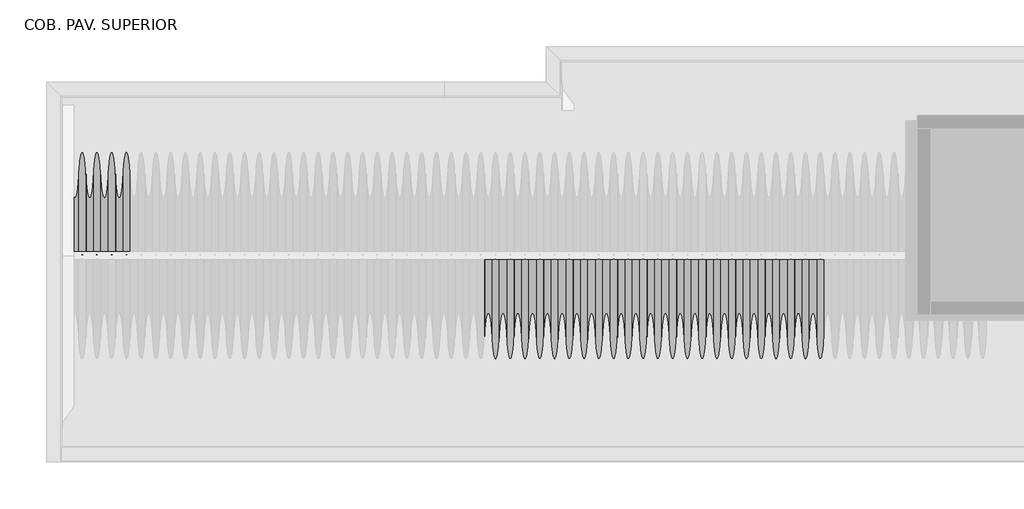
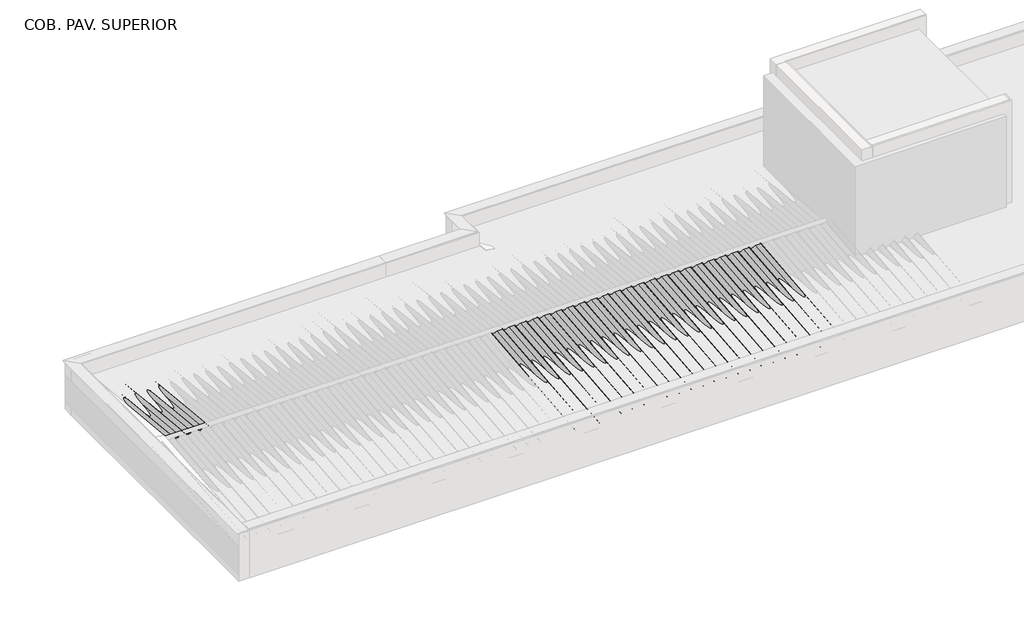
# One storey, part 3 of 8: 34 beams, 6 columns.
"""IFC4 building model written with IfcOpenShell, lengths in millimetres."""

import ifcopenshell
import ifcopenshell.guid

model = None  # the IFC model being written
_history = None  # IfcOwnerHistory: only IFC2X3 demands one
_inside = {}  # id of a spatial element -> (the spatial element, [elements in it])
_under = {}  # id of a project, library or spatial element -> (it, [spatial elements below it])
_declared = {}  # id of a project -> (the project, [libraries it declares])
_typed = {}  # id of a type object -> (the type object, [elements of that type])
_made_of = {}  # id of a material, layer set ... -> (it, [elements and type objects made of it])


def new_model(schema):
    """Start an empty IFC model of exactly this schema.

    Asked for "IFC4X3", IfcOpenShell would pick the latest addendum, in which some entities
    have other attributes; the version numbers below select the first issue.
    IFC2X3 requires an IfcOwnerHistory on every rooted entity: one is made here for all.
    """
    global model, _history
    if schema == "IFC4X3":
        model = ifcopenshell.file(schema_version=(4, 3, 0, 0))
    else:
        model = ifcopenshell.file(schema=schema)
    _inside.clear()
    _under.clear()
    _declared.clear()
    _typed.clear()
    _made_of.clear()
    _history = None
    if model.schema == "IFC2X3":
        org = make("IfcOrganization", Name="unknown")
        user = make(
            "IfcPersonAndOrganization",
            ThePerson=make("IfcPerson", FamilyName="unknown"),
            TheOrganization=org,
        )
        app = make(
            "IfcApplication",
            ApplicationDeveloper=org,
            Version="unknown",
            ApplicationFullName="unknown",
            ApplicationIdentifier="unknown",
        )
        _history = make(
            "IfcOwnerHistory",
            OwningUser=user,
            OwningApplication=app,
            ChangeAction="ADDED",
            CreationDate=0,
        )
    return model


def make(cls, **values):
    """One entity of the class cls with the attributes given. An attribute that is None is left unset."""
    return model.create_entity(
        cls, **{name: value for name, value in values.items() if value is not None}
    )


def rooted(cls, **values):
    """An entity with a GlobalId (a new one), such as an element, a storey or a relation."""
    return make(cls, GlobalId=ifcopenshell.guid.new(), OwnerHistory=_history, **values)


def si_unit(unit_type, name, prefix=None):
    """IfcSIUnit, for example si_unit("LENGTHUNIT", "METRE", prefix="MILLI")."""
    return make("IfcSIUnit", UnitType=unit_type, Prefix=prefix, Name=name)


def assignment(units):
    """IfcUnitAssignment: the units of a project."""
    return None if units is None else make("IfcUnitAssignment", Units=units)


def point(xyz):
    """IfcCartesianPoint."""
    return None if xyz is None else make("IfcCartesianPoint", Coordinates=xyz)


def direction(xyz):
    """IfcDirection."""
    return None if xyz is None else make("IfcDirection", DirectionRatios=xyz)


def frame(location, z_axis=None, x_axis=None):
    """IfcAxis2Placement3D, a coordinate frame: its origin and axes. An axis left out is left unset."""
    return make(
        "IfcAxis2Placement3D",
        Location=point(location),
        Axis=direction(z_axis),
        RefDirection=direction(x_axis),
    )


def frame_2d(location, x_axis=None):
    """IfcAxis2Placement2D, a coordinate frame in the plane: its origin and x axis."""
    return make(
        "IfcAxis2Placement2D", Location=point(location), RefDirection=direction(x_axis)
    )


def origin():
    """The frame at (0, 0, 0) with its axes left unset."""
    return frame((0.0, 0.0, 0.0))


def place(relative_to, where):
    """IfcLocalPlacement: puts the frame where relative to a parent placement (None: the world)."""
    return make(
        "IfcLocalPlacement", PlacementRelTo=relative_to, RelativePlacement=where
    )


def context(
    kind, dimensions, precision=None, world=None, true_north=None, identifier=None
):
    """IfcGeometricRepresentationContext, for example the 3D "Model" context."""
    return make(
        "IfcGeometricRepresentationContext",
        ContextIdentifier=identifier,
        ContextType=kind,
        CoordinateSpaceDimension=dimensions,
        Precision=precision,
        WorldCoordinateSystem=world,
        TrueNorth=true_north,
    )


def project(units=None, contexts=None):
    """IfcProject with its units and contexts."""
    return rooted(
        "IfcProject",
        Name="project",
        RepresentationContexts=contexts,
        UnitsInContext=assignment(units),
    )


def spatial(cls, under=None, at=None, **own):
    """A site, building, storey or space (cls), placed at a placement, below another one or the project."""
    s = rooted(cls, ObjectPlacement=at, **own)
    if under is not None:
        _under.setdefault(under.id(), (under, []))[1].append(s)
    return s


def polyline(points):
    """IfcPolyline through the points."""
    return make("IfcPolyline", Points=[point(p) for p in points])


def circle_curve(where, radius):
    """IfcCircle in the frame where."""
    return make("IfcCircle", Position=where, Radius=radius)


def trimmed(basis, trim1, trim2, sense, master):
    """IfcTrimmedCurve: the piece of a basis curve between two trims."""
    return make(
        "IfcTrimmedCurve",
        BasisCurve=basis,
        Trim1=trim1,
        Trim2=trim2,
        SenseAgreement=sense,
        MasterRepresentation=master,
    )


def segment(curve, same_sense, transition):
    """IfcCompositeCurveSegment."""
    return make(
        "IfcCompositeCurveSegment",
        Transition=transition,
        SameSense=same_sense,
        ParentCurve=curve,
    )


def composite_curve(segments, self_intersect=None):
    """IfcCompositeCurve: segments joined end to end."""
    return make("IfcCompositeCurve", Segments=segments, SelfIntersect=self_intersect)


def outline(outer, holes=None, kind="AREA"):
    """IfcArbitraryClosedProfileDef: a profile drawn as a closed curve; with holes, ...WithVoids."""
    if holes is None:
        return make("IfcArbitraryClosedProfileDef", ProfileType=kind, OuterCurve=outer)
    return make(
        "IfcArbitraryProfileDefWithVoids",
        ProfileType=kind,
        OuterCurve=outer,
        InnerCurves=holes,
    )


def extrude(swept, where, along, depth):
    """IfcExtrudedAreaSolid: the profile swept, set in the frame where, extruded along a direction by depth."""
    return make(
        "IfcExtrudedAreaSolid",
        SweptArea=swept,
        Position=where,
        ExtrudedDirection=direction(along),
        Depth=depth,
    )


def shape(context_of_items, identifier, shape_type, items):
    """IfcShapeRepresentation: the items that make up one representation, for example the "Body"."""
    return make(
        "IfcShapeRepresentation",
        ContextOfItems=context_of_items,
        RepresentationIdentifier=identifier,
        RepresentationType=shape_type,
        Items=items,
    )


def source(mapping_origin, context_of_items, identifier, shape_type, items):
    """IfcRepresentationMap: a shape defined once, which mapped items show again and again."""
    return make(
        "IfcRepresentationMap",
        MappingOrigin=mapping_origin,
        MappedRepresentation=shape(context_of_items, identifier, shape_type, items),
    )


def transform(
    local_origin,
    x_axis=None,
    y_axis=None,
    z_axis=None,
    scale=None,
    scale2=None,
    scale3=None,
    uniform=True,
):
    """IfcCartesianTransformationOperator3D, or its non-uniform kind. x_axis, y_axis, z_axis: its Axis1, 2, 3."""
    if uniform:
        return make(
            "IfcCartesianTransformationOperator3D",
            Axis1=direction(x_axis),
            Axis2=direction(y_axis),
            LocalOrigin=point(local_origin),
            Scale=scale,
            Axis3=direction(z_axis),
        )
    return make(
        "IfcCartesianTransformationOperator3DnonUniform",
        Axis1=direction(x_axis),
        Axis2=direction(y_axis),
        LocalOrigin=point(local_origin),
        Scale=scale,
        Axis3=direction(z_axis),
        Scale2=scale2,
        Scale3=scale3,
    )


def mapped(mapping_source, mapping_target):
    """IfcMappedItem: shows the shape of a source again, moved by a transform."""
    return make(
        "IfcMappedItem", MappingSource=mapping_source, MappingTarget=mapping_target
    )


def made_of(thing, what):
    """Note that an element or type object is made of a material, layer set ...; save() writes the relation."""
    if what is not None:
        _made_of.setdefault(what.id(), (what, []))[1].append(thing)
    return thing


def element(
    cls,
    number,
    at=None,
    inside=None,
    cuts=None,
    type_object=None,
    material=None,
    context=None,
    identifier="Body",
    shape_type=None,
    held_by="IfcProductDefinitionShape",
    body=None,
    shapes=None,
    **own,
):
    """One element of the class cls, such as IfcWall. Its Tag is "e" and its number.

    at: its placement. inside: the storey or other place that contains it. cuts: it is an
    opening in that element (IfcRelVoidsElement). A single representation is given by context,
    identifier, shape_type and body (its items); several are given by shapes. held_by: the class
    of the entity that holds the representations. save() writes the other relations.
    """
    e = rooted(cls, Tag="e%d" % number, ObjectPlacement=at, **own)
    if body is not None:
        shapes = [shape(context, identifier, shape_type, body)]
    if shapes is not None:
        e.Representation = make(held_by, Representations=shapes)
    if inside is not None:
        _inside.setdefault(inside.id(), (inside, []))[1].append(e)
    if cuts is not None:
        rooted(
            "IfcRelVoidsElement", RelatingBuildingElement=cuts, RelatedOpeningElement=e
        )
    if type_object is not None:
        _typed.setdefault(type_object.id(), (type_object, []))[1].append(e)
    return made_of(e, material)


def aggregate(whole, parts):
    """IfcRelAggregates: a whole, such as a stair, and the parts it consists of."""
    return rooted("IfcRelAggregates", RelatingObject=whole, RelatedObjects=parts)


def save(model, path):
    """Write the relations noted so far, then the file.

    IfcRelAggregates (storeys below a building ...), IfcRelContainedInSpatialStructure (elements
    in a storey), IfcRelDefinesByType, IfcRelAssociatesMaterial and IfcRelDeclares: one each for
    every whole, place, type object, material and project.
    """
    for whole, parts in _under.values():
        aggregate(whole, parts)
    for where, things in _inside.values():
        rooted(
            "IfcRelContainedInSpatialStructure",
            RelatedElements=things,
            RelatingStructure=where,
        )
    for kind, things in _typed.values():
        rooted("IfcRelDefinesByType", RelatedObjects=things, RelatingType=kind)
    for what, things in _made_of.values():
        rooted("IfcRelAssociatesMaterial", RelatedObjects=things, RelatingMaterial=what)
    for by, libraries in _declared.values():
        rooted("IfcRelDeclares", RelatingContext=by, RelatedDefinitions=libraries)
    model.write(path)


def beam_fe4ddbad(model_context):
    return source(origin(), model_context, "Body", "SweptSolid", [
        extrude(outline(polyline([(998.8971968, 30.0), (998.8971968, -30.0), (-998.8971974, -30.0), (-998.8971974, 30.0), (998.8971968, 30.0)])), frame((0.0, 0.0, -60.0), z_axis=(0.0, 0.0, 1.0), x_axis=(1.0, 0.0, 0.0)), (0.0, 0.0, 1.0), 120.0),
    ])


def column_6c15bf79(model_context):
    return source(origin(), model_context, "Body", "SweptSolid", [
        extrude(outline(polyline([(30.0, 80.0), (30.0, -80.0), (-30.0, -80.0), (-30.0, 80.0), (30.0, 80.0)])), frame((0.0, 0.0, 6710.0), z_axis=(0.0, 0.0, 1.0), x_axis=(1.0, 0.0, 0.0)), (0.0, 0.0, 1.0), 467.5),
    ])


def column_42eef9f8(model_context):
    return source(origin(), model_context, "Body", "SweptSolid", [
        extrude(outline(polyline([(30.0, 80.0), (30.0, -80.0), (-30.0, -80.0), (-30.0, 80.0), (30.0, 80.0)])), frame((0.0, 0.0, 6710.0), z_axis=(0.0, 0.0, 1.0), x_axis=(1.0, 0.0, 0.0)), (0.0, 0.0, 1.0), 227.1),
    ])


model = new_model("IFC4")

# Units and contexts
model_context = context("Model", 3, world=origin())
ifc_project = project(units=[si_unit("LENGTHUNIT", "METRE", prefix="MILLI")], contexts=[model_context])

# Site, building, storey
site = spatial("IfcSite", under=ifc_project)
building = spatial("IfcBuilding", under=site)
storey = spatial("IfcBuildingStorey", under=building, Name="COB. PAV. SUPERIOR", Elevation=6650.0)

# Beams
placement = place(None, origin())
beam_shape = beam_fe4ddbad(model_context)
element("IfcBeam", 1, ObjectType="Madeira de lei : Berço 6x12cm", at=placement, inside=storey, context=model_context, shape_type="MappedRepresentation", body=[
    mapped(beam_shape, transform((-11738.1841096, -7777.6209418, 6680.0), x_axis=(1.0, 0.0, 0.0), y_axis=(0.0, 0.0, -1.0), z_axis=(0.0, 1.0, 0.0))),
])
element("IfcBeam", 2, ObjectType="Madeira de lei : Berço 6x12cm", at=placement, inside=storey, context=model_context, shape_type="MappedRepresentation", body=[
    mapped(beam_shape, transform((-5744.8009251, -9189.768869, 6680.0), x_axis=(1.0, 0.0, 0.0), y_axis=(0.0, 0.0, -1.0), z_axis=(0.0, 1.0, 0.0))),
])
element("IfcBeam", 3, ObjectType="Madeira de lei : Berço 6x12cm", at=placement, inside=storey, context=model_context, shape_type="MappedRepresentation", body=[
    mapped(beam_shape, transform((-3747.0065303, -9189.768869, 6680.0), x_axis=(1.0, 0.0, 0.0), y_axis=(0.0, 0.0, -1.0), z_axis=(0.0, 1.0, 0.0))),
])
element("IfcBeam", 4, ObjectType="Madeira de lei : Berço 6x12cm", at=placement, inside=storey, context=model_context, shape_type="MappedRepresentation", body=[
    mapped(beam_shape, transform((-1749.2121355, -9189.768869, 6680.0), x_axis=(1.0, 0.0, 0.0), y_axis=(0.0, 0.0, -1.0), z_axis=(0.0, 1.0, 0.0))),
])
element("IfcBeam", 5, ObjectType="Madeira de lei : Berço 6x12cm", at=placement, inside=storey, context=model_context, shape_type="MappedRepresentation", body=[
    mapped(beam_shape, transform((-3747.0065303, -10631.818869, 6680.0), x_axis=(1.0, 0.0, 0.0), y_axis=(0.0, 0.0, -1.0), z_axis=(0.0, 1.0, 0.0))),
])
element("IfcBeam", 6, ObjectType="Madeira de lei : Berço 6x12cm", at=placement, inside=storey, context=model_context, shape_type="MappedRepresentation", body=[
    mapped(beam_shape, transform((-1749.2121355, -10631.818869, 6680.0), x_axis=(1.0, 0.0, 0.0), y_axis=(0.0, 0.0, -1.0), z_axis=(0.0, 1.0, 0.0))),
])
element("IfcBeam", 7, ObjectType="Telha Ondulada : Fibrocimento", at=placement, inside=storey, context=model_context, shape_type="SweptSolid", body=[
    extrude(outline(composite_curve([segment(trimmed(circle_curve(frame_2d((0.0, 66.7939461)), 66.7939461), [point((29.3501489, 6.7939461))], [point((29.3501489, 126.7939461))], True, "CARTESIAN"), True, "CONTINUOUS"), segment(polyline([(29.3501489, 126.7939461), (31.5472154, 131.2853711)]), True, "CONTINUOUS"), segment(trimmed(circle_curve(frame_2d((0.0, 66.7939461)), 71.7939461), [point((31.5472154, 131.2853711))], [point((31.5472154, 2.3025211))], False, "CARTESIAN"), True, "CONTINUOUS"), segment(trimmed(circle_curve(frame_2d((58.7002978, -53.2060539)), 61.7939461), [point((31.5472154, 2.3025211))], [point((31.5472154, -108.7146289))], True, "CARTESIAN"), True, "CONTINUOUS"), segment(polyline([(31.5472154, -108.7146289), (29.3501489, -113.2060539)]), True, "CONTINUOUS"), segment(trimmed(circle_curve(frame_2d((58.7002978, -53.2060539)), 66.7939461), [point((29.3501489, -113.2060539))], [point((29.3501489, 6.7939461))], False, "CARTESIAN"), True, "CONTINUOUS")], self_intersect=False)), frame((-5606.7843743, -10831.9594023, 7106.8215886), z_axis=(0.0, 0.9950371902099894, 0.09950371902099749), x_axis=(0.0, 0.09950371902099749, -0.9950371902099894)), (0.0, 0.0, 1.0), 3060.4439799),
])
element("IfcBeam", 8, ObjectType="Telha Ondulada : Fibrocimento", at=placement, inside=storey, context=model_context, shape_type="SweptSolid", body=[
    extrude(outline(composite_curve([segment(trimmed(circle_curve(frame_2d((0.0, 66.7939461)), 66.7939461), [point((29.3501489, 6.7939461))], [point((29.3501489, 126.7939461))], True, "CARTESIAN"), True, "CONTINUOUS"), segment(polyline([(29.3501489, 126.7939461), (31.5472154, 131.2853711)]), True, "CONTINUOUS"), segment(trimmed(circle_curve(frame_2d((0.0, 66.7939461)), 71.7939461), [point((31.5472154, 131.2853711))], [point((31.5472154, 2.3025211))], False, "CARTESIAN"), True, "CONTINUOUS"), segment(trimmed(circle_curve(frame_2d((58.7002978, -53.2060539)), 61.7939461), [point((31.5472154, 2.3025211))], [point((31.5472154, -108.7146289))], True, "CARTESIAN"), True, "CONTINUOUS"), segment(polyline([(31.5472154, -108.7146289), (29.3501489, -113.2060539)]), True, "CONTINUOUS"), segment(trimmed(circle_curve(frame_2d((58.7002978, -53.2060539)), 66.7939461), [point((29.3501489, -113.2060539))], [point((29.3501489, 6.7939461))], False, "CARTESIAN"), True, "CONTINUOUS")], self_intersect=False)), frame((-5362.2843743, -10831.9594023, 7106.8215886), z_axis=(0.0, 0.9950371902099894, 0.09950371902099749), x_axis=(0.0, 0.09950371902099749, -0.9950371902099894)), (0.0, 0.0, 1.0), 3060.4439799),
])
element("IfcBeam", 9, ObjectType="Telha Ondulada : Fibrocimento", at=placement, inside=storey, context=model_context, shape_type="SweptSolid", body=[
    extrude(outline(composite_curve([segment(trimmed(circle_curve(frame_2d((0.0, 66.7939461)), 66.7939461), [point((29.3501489, 6.7939461))], [point((29.3501489, 126.7939461))], True, "CARTESIAN"), True, "CONTINUOUS"), segment(polyline([(29.3501489, 126.7939461), (31.5472154, 131.2853711)]), True, "CONTINUOUS"), segment(trimmed(circle_curve(frame_2d((0.0, 66.7939461)), 71.7939461), [point((31.5472154, 131.2853711))], [point((31.5472154, 2.3025211))], False, "CARTESIAN"), True, "CONTINUOUS"), segment(trimmed(circle_curve(frame_2d((58.7002978, -53.2060539)), 61.7939461), [point((31.5472154, 2.3025211))], [point((31.5472154, -108.7146289))], True, "CARTESIAN"), True, "CONTINUOUS"), segment(polyline([(31.5472154, -108.7146289), (29.3501489, -113.2060539)]), True, "CONTINUOUS"), segment(trimmed(circle_curve(frame_2d((58.7002978, -53.2060539)), 66.7939461), [point((29.3501489, -113.2060539))], [point((29.3501489, 6.7939461))], False, "CARTESIAN"), True, "CONTINUOUS")], self_intersect=False)), frame((-5117.7843743, -10831.9594023, 7106.8215886), z_axis=(0.0, 0.9950371902099894, 0.09950371902099749), x_axis=(0.0, 0.09950371902099749, -0.9950371902099894)), (0.0, 0.0, 1.0), 3060.4439799),
])
element("IfcBeam", 10, ObjectType="Telha Ondulada : Fibrocimento", at=placement, inside=storey, context=model_context, shape_type="SweptSolid", body=[
    extrude(outline(composite_curve([segment(trimmed(circle_curve(frame_2d((0.0, 66.7939461)), 66.7939461), [point((29.3501489, 6.7939461))], [point((29.3501489, 126.7939461))], True, "CARTESIAN"), True, "CONTINUOUS"), segment(polyline([(29.3501489, 126.7939461), (31.5472154, 131.2853711)]), True, "CONTINUOUS"), segment(trimmed(circle_curve(frame_2d((0.0, 66.7939461)), 71.7939461), [point((31.5472154, 131.2853711))], [point((31.5472154, 2.3025211))], False, "CARTESIAN"), True, "CONTINUOUS"), segment(trimmed(circle_curve(frame_2d((58.7002978, -53.2060539)), 61.7939461), [point((31.5472154, 2.3025211))], [point((31.5472154, -108.7146289))], True, "CARTESIAN"), True, "CONTINUOUS"), segment(polyline([(31.5472154, -108.7146289), (29.3501489, -113.2060539)]), True, "CONTINUOUS"), segment(trimmed(circle_curve(frame_2d((58.7002978, -53.2060539)), 66.7939461), [point((29.3501489, -113.2060539))], [point((29.3501489, 6.7939461))], False, "CARTESIAN"), True, "CONTINUOUS")], self_intersect=False)), frame((-4873.2843743, -10831.9594023, 7106.8215886), z_axis=(0.0, 0.9950371902099894, 0.09950371902099749), x_axis=(0.0, 0.09950371902099749, -0.9950371902099894)), (0.0, 0.0, 1.0), 3060.4439799),
])
element("IfcBeam", 11, ObjectType="Telha Ondulada : Fibrocimento", at=placement, inside=storey, context=model_context, shape_type="SweptSolid", body=[
    extrude(outline(composite_curve([segment(trimmed(circle_curve(frame_2d((0.0, 66.7939461)), 66.7939461), [point((29.3501489, 6.7939461))], [point((29.3501489, 126.7939461))], True, "CARTESIAN"), True, "CONTINUOUS"), segment(polyline([(29.3501489, 126.7939461), (31.5472154, 131.2853711)]), True, "CONTINUOUS"), segment(trimmed(circle_curve(frame_2d((0.0, 66.7939461)), 71.7939461), [point((31.5472154, 131.2853711))], [point((31.5472154, 2.3025211))], False, "CARTESIAN"), True, "CONTINUOUS"), segment(trimmed(circle_curve(frame_2d((58.7002978, -53.2060539)), 61.7939461), [point((31.5472154, 2.3025211))], [point((31.5472154, -108.7146289))], True, "CARTESIAN"), True, "CONTINUOUS"), segment(polyline([(31.5472154, -108.7146289), (29.3501489, -113.2060539)]), True, "CONTINUOUS"), segment(trimmed(circle_curve(frame_2d((58.7002978, -53.2060539)), 66.7939461), [point((29.3501489, -113.2060539))], [point((29.3501489, 6.7939461))], False, "CARTESIAN"), True, "CONTINUOUS")], self_intersect=False)), frame((-4628.7843743, -10831.9594023, 7106.8215886), z_axis=(0.0, 0.9950371902099894, 0.09950371902099749), x_axis=(0.0, 0.09950371902099749, -0.9950371902099894)), (0.0, 0.0, 1.0), 3060.4439799),
])
element("IfcBeam", 12, ObjectType="Telha Ondulada : Fibrocimento", at=placement, inside=storey, context=model_context, shape_type="SweptSolid", body=[
    extrude(outline(composite_curve([segment(trimmed(circle_curve(frame_2d((0.0, 66.7939461)), 66.7939461), [point((29.3501489, 6.7939461))], [point((29.3501489, 126.7939461))], True, "CARTESIAN"), True, "CONTINUOUS"), segment(polyline([(29.3501489, 126.7939461), (31.5472154, 131.2853711)]), True, "CONTINUOUS"), segment(trimmed(circle_curve(frame_2d((0.0, 66.7939461)), 71.7939461), [point((31.5472154, 131.2853711))], [point((31.5472154, 2.3025211))], False, "CARTESIAN"), True, "CONTINUOUS"), segment(trimmed(circle_curve(frame_2d((58.7002978, -53.2060539)), 61.7939461), [point((31.5472154, 2.3025211))], [point((31.5472154, -108.7146289))], True, "CARTESIAN"), True, "CONTINUOUS"), segment(polyline([(31.5472154, -108.7146289), (29.3501489, -113.2060539)]), True, "CONTINUOUS"), segment(trimmed(circle_curve(frame_2d((58.7002978, -53.2060539)), 66.7939461), [point((29.3501489, -113.2060539))], [point((29.3501489, 6.7939461))], False, "CARTESIAN"), True, "CONTINUOUS")], self_intersect=False)), frame((-4384.2843743, -10831.9594023, 7106.8215886), z_axis=(0.0, 0.9950371902099894, 0.09950371902099749), x_axis=(0.0, 0.09950371902099749, -0.9950371902099894)), (0.0, 0.0, 1.0), 3060.4439799),
])
element("IfcBeam", 13, ObjectType="Telha Ondulada : Fibrocimento", at=placement, inside=storey, context=model_context, shape_type="SweptSolid", body=[
    extrude(outline(composite_curve([segment(trimmed(circle_curve(frame_2d((0.0, 66.7939461)), 66.7939461), [point((29.3501489, 6.7939461))], [point((29.3501489, 126.7939461))], True, "CARTESIAN"), True, "CONTINUOUS"), segment(polyline([(29.3501489, 126.7939461), (31.5472154, 131.2853711)]), True, "CONTINUOUS"), segment(trimmed(circle_curve(frame_2d((0.0, 66.7939461)), 71.7939461), [point((31.5472154, 131.2853711))], [point((31.5472154, 2.3025211))], False, "CARTESIAN"), True, "CONTINUOUS"), segment(trimmed(circle_curve(frame_2d((58.7002978, -53.2060539)), 61.7939461), [point((31.5472154, 2.3025211))], [point((31.5472154, -108.7146289))], True, "CARTESIAN"), True, "CONTINUOUS"), segment(polyline([(31.5472154, -108.7146289), (29.3501489, -113.2060539)]), True, "CONTINUOUS"), segment(trimmed(circle_curve(frame_2d((58.7002978, -53.2060539)), 66.7939461), [point((29.3501489, -113.2060539))], [point((29.3501489, 6.7939461))], False, "CARTESIAN"), True, "CONTINUOUS")], self_intersect=False)), frame((-4139.7843743, -10831.9594023, 7106.8215886), z_axis=(0.0, 0.9950371902099894, 0.09950371902099749), x_axis=(0.0, 0.09950371902099749, -0.9950371902099894)), (0.0, 0.0, 1.0), 3060.4439799),
])
element("IfcBeam", 14, ObjectType="Telha Ondulada : Fibrocimento", at=placement, inside=storey, context=model_context, shape_type="SweptSolid", body=[
    extrude(outline(composite_curve([segment(trimmed(circle_curve(frame_2d((0.0, 66.7939461)), 66.7939461), [point((29.3501489, 6.7939461))], [point((29.3501489, 126.7939461))], True, "CARTESIAN"), True, "CONTINUOUS"), segment(polyline([(29.3501489, 126.7939461), (31.5472154, 131.2853711)]), True, "CONTINUOUS"), segment(trimmed(circle_curve(frame_2d((0.0, 66.7939461)), 71.7939461), [point((31.5472154, 131.2853711))], [point((31.5472154, 2.3025211))], False, "CARTESIAN"), True, "CONTINUOUS"), segment(trimmed(circle_curve(frame_2d((58.7002978, -53.2060539)), 61.7939461), [point((31.5472154, 2.3025211))], [point((31.5472154, -108.7146289))], True, "CARTESIAN"), True, "CONTINUOUS"), segment(polyline([(31.5472154, -108.7146289), (29.3501489, -113.2060539)]), True, "CONTINUOUS"), segment(trimmed(circle_curve(frame_2d((58.7002978, -53.2060539)), 66.7939461), [point((29.3501489, -113.2060539))], [point((29.3501489, 6.7939461))], False, "CARTESIAN"), True, "CONTINUOUS")], self_intersect=False)), frame((-3895.2843743, -10831.9594023, 7106.8215886), z_axis=(0.0, 0.9950371902099894, 0.09950371902099749), x_axis=(0.0, 0.09950371902099749, -0.9950371902099894)), (0.0, 0.0, 1.0), 3060.4439799),
])
element("IfcBeam", 15, ObjectType="Telha Ondulada : Fibrocimento", at=placement, inside=storey, context=model_context, shape_type="SweptSolid", body=[
    extrude(outline(composite_curve([segment(trimmed(circle_curve(frame_2d((0.0, 66.7939461)), 66.7939461), [point((29.3501489, 6.7939461))], [point((29.3501489, 126.7939461))], True, "CARTESIAN"), True, "CONTINUOUS"), segment(polyline([(29.3501489, 126.7939461), (31.5472154, 131.2853711)]), True, "CONTINUOUS"), segment(trimmed(circle_curve(frame_2d((0.0, 66.7939461)), 71.7939461), [point((31.5472154, 131.2853711))], [point((31.5472154, 2.3025211))], False, "CARTESIAN"), True, "CONTINUOUS"), segment(trimmed(circle_curve(frame_2d((58.7002978, -53.2060539)), 61.7939461), [point((31.5472154, 2.3025211))], [point((31.5472154, -108.7146289))], True, "CARTESIAN"), True, "CONTINUOUS"), segment(polyline([(31.5472154, -108.7146289), (29.3501489, -113.2060539)]), True, "CONTINUOUS"), segment(trimmed(circle_curve(frame_2d((58.7002978, -53.2060539)), 66.7939461), [point((29.3501489, -113.2060539))], [point((29.3501489, 6.7939461))], False, "CARTESIAN"), True, "CONTINUOUS")], self_intersect=False)), frame((-3650.7843743, -10831.9594023, 7106.8215886), z_axis=(0.0, 0.9950371902099894, 0.09950371902099749), x_axis=(0.0, 0.09950371902099749, -0.9950371902099894)), (0.0, 0.0, 1.0), 3060.4439799),
])
element("IfcBeam", 16, ObjectType="Telha Ondulada : Fibrocimento", at=placement, inside=storey, context=model_context, shape_type="SweptSolid", body=[
    extrude(outline(composite_curve([segment(trimmed(circle_curve(frame_2d((0.0, 66.7939461)), 66.7939461), [point((29.3501489, 6.7939461))], [point((29.3501489, 126.7939461))], True, "CARTESIAN"), True, "CONTINUOUS"), segment(polyline([(29.3501489, 126.7939461), (31.5472154, 131.2853711)]), True, "CONTINUOUS"), segment(trimmed(circle_curve(frame_2d((0.0, 66.7939461)), 71.7939461), [point((31.5472154, 131.2853711))], [point((31.5472154, 2.3025211))], False, "CARTESIAN"), True, "CONTINUOUS"), segment(trimmed(circle_curve(frame_2d((58.7002978, -53.2060539)), 61.7939461), [point((31.5472154, 2.3025211))], [point((31.5472154, -108.7146289))], True, "CARTESIAN"), True, "CONTINUOUS"), segment(polyline([(31.5472154, -108.7146289), (29.3501489, -113.2060539)]), True, "CONTINUOUS"), segment(trimmed(circle_curve(frame_2d((58.7002978, -53.2060539)), 66.7939461), [point((29.3501489, -113.2060539))], [point((29.3501489, 6.7939461))], False, "CARTESIAN"), True, "CONTINUOUS")], self_intersect=False)), frame((-3406.2843743, -10831.9594023, 7106.8215886), z_axis=(0.0, 0.9950371902099894, 0.09950371902099749), x_axis=(0.0, 0.09950371902099749, -0.9950371902099894)), (0.0, 0.0, 1.0), 3060.4439799),
])
element("IfcBeam", 17, ObjectType="Telha Ondulada : Fibrocimento", at=placement, inside=storey, context=model_context, shape_type="SweptSolid", body=[
    extrude(outline(composite_curve([segment(trimmed(circle_curve(frame_2d((0.0, 66.7939461)), 66.7939461), [point((29.3501489, 6.7939461))], [point((29.3501489, 126.7939461))], True, "CARTESIAN"), True, "CONTINUOUS"), segment(polyline([(29.3501489, 126.7939461), (31.5472154, 131.2853711)]), True, "CONTINUOUS"), segment(trimmed(circle_curve(frame_2d((0.0, 66.7939461)), 71.7939461), [point((31.5472154, 131.2853711))], [point((31.5472154, 2.3025211))], False, "CARTESIAN"), True, "CONTINUOUS"), segment(trimmed(circle_curve(frame_2d((58.7002978, -53.2060539)), 61.7939461), [point((31.5472154, 2.3025211))], [point((31.5472154, -108.7146289))], True, "CARTESIAN"), True, "CONTINUOUS"), segment(polyline([(31.5472154, -108.7146289), (29.3501489, -113.2060539)]), True, "CONTINUOUS"), segment(trimmed(circle_curve(frame_2d((58.7002978, -53.2060539)), 66.7939461), [point((29.3501489, -113.2060539))], [point((29.3501489, 6.7939461))], False, "CARTESIAN"), True, "CONTINUOUS")], self_intersect=False)), frame((-3161.7843743, -10831.9594023, 7106.8215886), z_axis=(0.0, 0.9950371902099894, 0.09950371902099749), x_axis=(0.0, 0.09950371902099749, -0.9950371902099894)), (0.0, 0.0, 1.0), 3060.4439799),
])
element("IfcBeam", 18, ObjectType="Telha Ondulada : Fibrocimento", at=placement, inside=storey, context=model_context, shape_type="SweptSolid", body=[
    extrude(outline(composite_curve([segment(trimmed(circle_curve(frame_2d((0.0, 66.7939461)), 66.7939461), [point((29.3501489, 6.7939461))], [point((29.3501489, 126.7939461))], True, "CARTESIAN"), True, "CONTINUOUS"), segment(polyline([(29.3501489, 126.7939461), (31.5472154, 131.2853711)]), True, "CONTINUOUS"), segment(trimmed(circle_curve(frame_2d((0.0, 66.7939461)), 71.7939461), [point((31.5472154, 131.2853711))], [point((31.5472154, 2.3025211))], False, "CARTESIAN"), True, "CONTINUOUS"), segment(trimmed(circle_curve(frame_2d((58.7002978, -53.2060539)), 61.7939461), [point((31.5472154, 2.3025211))], [point((31.5472154, -108.7146289))], True, "CARTESIAN"), True, "CONTINUOUS"), segment(polyline([(31.5472154, -108.7146289), (29.3501489, -113.2060539)]), True, "CONTINUOUS"), segment(trimmed(circle_curve(frame_2d((58.7002978, -53.2060539)), 66.7939461), [point((29.3501489, -113.2060539))], [point((29.3501489, 6.7939461))], False, "CARTESIAN"), True, "CONTINUOUS")], self_intersect=False)), frame((-2917.2843743, -10831.9594023, 7106.8215886), z_axis=(0.0, 0.9950371902099894, 0.09950371902099749), x_axis=(0.0, 0.09950371902099749, -0.9950371902099894)), (0.0, 0.0, 1.0), 3060.4439799),
])
element("IfcBeam", 19, ObjectType="Telha Ondulada : Fibrocimento", at=placement, inside=storey, context=model_context, shape_type="SweptSolid", body=[
    extrude(outline(composite_curve([segment(trimmed(circle_curve(frame_2d((0.0, 66.7939461)), 66.7939461), [point((29.3501489, 6.7939461))], [point((29.3501489, 126.7939461))], True, "CARTESIAN"), True, "CONTINUOUS"), segment(polyline([(29.3501489, 126.7939461), (31.5472154, 131.2853711)]), True, "CONTINUOUS"), segment(trimmed(circle_curve(frame_2d((0.0, 66.7939461)), 71.7939461), [point((31.5472154, 131.2853711))], [point((31.5472154, 2.3025211))], False, "CARTESIAN"), True, "CONTINUOUS"), segment(trimmed(circle_curve(frame_2d((58.7002978, -53.2060539)), 61.7939461), [point((31.5472154, 2.3025211))], [point((31.5472154, -108.7146289))], True, "CARTESIAN"), True, "CONTINUOUS"), segment(polyline([(31.5472154, -108.7146289), (29.3501489, -113.2060539)]), True, "CONTINUOUS"), segment(trimmed(circle_curve(frame_2d((58.7002978, -53.2060539)), 66.7939461), [point((29.3501489, -113.2060539))], [point((29.3501489, 6.7939461))], False, "CARTESIAN"), True, "CONTINUOUS")], self_intersect=False)), frame((-2672.7843743, -10831.9594023, 7106.8215886), z_axis=(0.0, 0.9950371902099894, 0.09950371902099749), x_axis=(0.0, 0.09950371902099749, -0.9950371902099894)), (0.0, 0.0, 1.0), 3060.4439799),
])
element("IfcBeam", 20, ObjectType="Telha Ondulada : Fibrocimento", at=placement, inside=storey, context=model_context, shape_type="SweptSolid", body=[
    extrude(outline(composite_curve([segment(trimmed(circle_curve(frame_2d((0.0, 66.7939461)), 66.7939461), [point((29.3501489, 6.7939461))], [point((29.3501489, 126.7939461))], True, "CARTESIAN"), True, "CONTINUOUS"), segment(polyline([(29.3501489, 126.7939461), (31.5472154, 131.2853711)]), True, "CONTINUOUS"), segment(trimmed(circle_curve(frame_2d((0.0, 66.7939461)), 71.7939461), [point((31.5472154, 131.2853711))], [point((31.5472154, 2.3025211))], False, "CARTESIAN"), True, "CONTINUOUS"), segment(trimmed(circle_curve(frame_2d((58.7002978, -53.2060539)), 61.7939461), [point((31.5472154, 2.3025211))], [point((31.5472154, -108.7146289))], True, "CARTESIAN"), True, "CONTINUOUS"), segment(polyline([(31.5472154, -108.7146289), (29.3501489, -113.2060539)]), True, "CONTINUOUS"), segment(trimmed(circle_curve(frame_2d((58.7002978, -53.2060539)), 66.7939461), [point((29.3501489, -113.2060539))], [point((29.3501489, 6.7939461))], False, "CARTESIAN"), True, "CONTINUOUS")], self_intersect=False)), frame((-2428.2843743, -10831.9594023, 7106.8215886), z_axis=(0.0, 0.9950371902099894, 0.09950371902099749), x_axis=(0.0, 0.09950371902099749, -0.9950371902099894)), (0.0, 0.0, 1.0), 3060.4439799),
])
element("IfcBeam", 21, ObjectType="Telha Ondulada : Fibrocimento", at=placement, inside=storey, context=model_context, shape_type="SweptSolid", body=[
    extrude(outline(composite_curve([segment(trimmed(circle_curve(frame_2d((0.0, 66.7939461)), 66.7939461), [point((29.3501489, 6.7939461))], [point((29.3501489, 126.7939461))], True, "CARTESIAN"), True, "CONTINUOUS"), segment(polyline([(29.3501489, 126.7939461), (31.5472154, 131.2853711)]), True, "CONTINUOUS"), segment(trimmed(circle_curve(frame_2d((0.0, 66.7939461)), 71.7939461), [point((31.5472154, 131.2853711))], [point((31.5472154, 2.3025211))], False, "CARTESIAN"), True, "CONTINUOUS"), segment(trimmed(circle_curve(frame_2d((58.7002978, -53.2060539)), 61.7939461), [point((31.5472154, 2.3025211))], [point((31.5472154, -108.7146289))], True, "CARTESIAN"), True, "CONTINUOUS"), segment(polyline([(31.5472154, -108.7146289), (29.3501489, -113.2060539)]), True, "CONTINUOUS"), segment(trimmed(circle_curve(frame_2d((58.7002978, -53.2060539)), 66.7939461), [point((29.3501489, -113.2060539))], [point((29.3501489, 6.7939461))], False, "CARTESIAN"), True, "CONTINUOUS")], self_intersect=False)), frame((-2183.7843743, -10831.9594023, 7106.8215886), z_axis=(0.0, 0.9950371902099894, 0.09950371902099749), x_axis=(0.0, 0.09950371902099749, -0.9950371902099894)), (0.0, 0.0, 1.0), 3060.4439799),
])
element("IfcBeam", 22, ObjectType="Telha Ondulada : Fibrocimento", at=placement, inside=storey, context=model_context, shape_type="SweptSolid", body=[
    extrude(outline(composite_curve([segment(trimmed(circle_curve(frame_2d((0.0, 66.7939461)), 66.7939461), [point((29.3501489, 6.7939461))], [point((29.3501489, 126.7939461))], True, "CARTESIAN"), True, "CONTINUOUS"), segment(polyline([(29.3501489, 126.7939461), (31.5472154, 131.2853711)]), True, "CONTINUOUS"), segment(trimmed(circle_curve(frame_2d((0.0, 66.7939461)), 71.7939461), [point((31.5472154, 131.2853711))], [point((31.5472154, 2.3025211))], False, "CARTESIAN"), True, "CONTINUOUS"), segment(trimmed(circle_curve(frame_2d((58.7002978, -53.2060539)), 61.7939461), [point((31.5472154, 2.3025211))], [point((31.5472154, -108.7146289))], True, "CARTESIAN"), True, "CONTINUOUS"), segment(polyline([(31.5472154, -108.7146289), (29.3501489, -113.2060539)]), True, "CONTINUOUS"), segment(trimmed(circle_curve(frame_2d((58.7002978, -53.2060539)), 66.7939461), [point((29.3501489, -113.2060539))], [point((29.3501489, 6.7939461))], False, "CARTESIAN"), True, "CONTINUOUS")], self_intersect=False)), frame((-1939.2843743, -10831.9594023, 7106.8215886), z_axis=(0.0, 0.9950371902099894, 0.09950371902099749), x_axis=(0.0, 0.09950371902099749, -0.9950371902099894)), (0.0, 0.0, 1.0), 3060.4439799),
])
element("IfcBeam", 23, ObjectType="Telha Ondulada : Fibrocimento", at=placement, inside=storey, context=model_context, shape_type="SweptSolid", body=[
    extrude(outline(composite_curve([segment(trimmed(circle_curve(frame_2d((0.0, 66.7939461)), 66.7939461), [point((29.3501489, 6.7939461))], [point((29.3501489, 126.7939461))], True, "CARTESIAN"), True, "CONTINUOUS"), segment(polyline([(29.3501489, 126.7939461), (31.5472154, 131.2853711)]), True, "CONTINUOUS"), segment(trimmed(circle_curve(frame_2d((0.0, 66.7939461)), 71.7939461), [point((31.5472154, 131.2853711))], [point((31.5472154, 2.3025211))], False, "CARTESIAN"), True, "CONTINUOUS"), segment(trimmed(circle_curve(frame_2d((58.7002978, -53.2060539)), 61.7939461), [point((31.5472154, 2.3025211))], [point((31.5472154, -108.7146289))], True, "CARTESIAN"), True, "CONTINUOUS"), segment(polyline([(31.5472154, -108.7146289), (29.3501489, -113.2060539)]), True, "CONTINUOUS"), segment(trimmed(circle_curve(frame_2d((58.7002978, -53.2060539)), 66.7939461), [point((29.3501489, -113.2060539))], [point((29.3501489, 6.7939461))], False, "CARTESIAN"), True, "CONTINUOUS")], self_intersect=False)), frame((-1694.7843743, -10831.9594023, 7106.8215886), z_axis=(0.0, 0.9950371902099894, 0.09950371902099749), x_axis=(0.0, 0.09950371902099749, -0.9950371902099894)), (0.0, 0.0, 1.0), 3060.4439799),
])
element("IfcBeam", 24, ObjectType="Telha Ondulada : Fibrocimento", at=placement, inside=storey, context=model_context, shape_type="SweptSolid", body=[
    extrude(outline(composite_curve([segment(trimmed(circle_curve(frame_2d((0.0, 66.7939461)), 66.7939461), [point((29.3501489, 6.7939461))], [point((29.3501489, 126.7939461))], True, "CARTESIAN"), True, "CONTINUOUS"), segment(polyline([(29.3501489, 126.7939461), (31.5472154, 131.2853711)]), True, "CONTINUOUS"), segment(trimmed(circle_curve(frame_2d((0.0, 66.7939461)), 71.7939461), [point((31.5472154, 131.2853711))], [point((31.5472154, 2.3025211))], False, "CARTESIAN"), True, "CONTINUOUS"), segment(trimmed(circle_curve(frame_2d((58.7002978, -53.2060539)), 61.7939461), [point((31.5472154, 2.3025211))], [point((31.5472154, -108.7146289))], True, "CARTESIAN"), True, "CONTINUOUS"), segment(polyline([(31.5472154, -108.7146289), (29.3501489, -113.2060539)]), True, "CONTINUOUS"), segment(trimmed(circle_curve(frame_2d((58.7002978, -53.2060539)), 66.7939461), [point((29.3501489, -113.2060539))], [point((29.3501489, 6.7939461))], False, "CARTESIAN"), True, "CONTINUOUS")], self_intersect=False)), frame((-1450.2843743, -10831.9594023, 7106.8215886), z_axis=(0.0, 0.9950371902099894, 0.09950371902099749), x_axis=(0.0, 0.09950371902099749, -0.9950371902099894)), (0.0, 0.0, 1.0), 3060.4439799),
])
element("IfcBeam", 25, ObjectType="Telha Ondulada : Fibrocimento", at=placement, inside=storey, context=model_context, shape_type="SweptSolid", body=[
    extrude(outline(composite_curve([segment(trimmed(circle_curve(frame_2d((0.0, 66.7939461)), 66.7939461), [point((29.3501489, 6.7939461))], [point((29.3501489, 126.7939461))], True, "CARTESIAN"), True, "CONTINUOUS"), segment(polyline([(29.3501489, 126.7939461), (31.5472154, 131.2853711)]), True, "CONTINUOUS"), segment(trimmed(circle_curve(frame_2d((0.0, 66.7939461)), 71.7939461), [point((31.5472154, 131.2853711))], [point((31.5472154, 2.3025211))], False, "CARTESIAN"), True, "CONTINUOUS"), segment(trimmed(circle_curve(frame_2d((58.7002978, -53.2060539)), 61.7939461), [point((31.5472154, 2.3025211))], [point((31.5472154, -108.7146289))], True, "CARTESIAN"), True, "CONTINUOUS"), segment(polyline([(31.5472154, -108.7146289), (29.3501489, -113.2060539)]), True, "CONTINUOUS"), segment(trimmed(circle_curve(frame_2d((58.7002978, -53.2060539)), 66.7939461), [point((29.3501489, -113.2060539))], [point((29.3501489, 6.7939461))], False, "CARTESIAN"), True, "CONTINUOUS")], self_intersect=False)), frame((-1205.7843743, -10831.9594023, 7106.8215886), z_axis=(0.0, 0.9950371902099894, 0.09950371902099749), x_axis=(0.0, 0.09950371902099749, -0.9950371902099894)), (0.0, 0.0, 1.0), 3060.4439799),
])
element("IfcBeam", 26, ObjectType="Telha Ondulada : Fibrocimento", at=placement, inside=storey, context=model_context, shape_type="SweptSolid", body=[
    extrude(outline(composite_curve([segment(trimmed(circle_curve(frame_2d((0.0, 66.7939461)), 66.7939461), [point((29.3501489, 6.7939461))], [point((29.3501489, 126.7939461))], True, "CARTESIAN"), True, "CONTINUOUS"), segment(polyline([(29.3501489, 126.7939461), (31.5472154, 131.2853711)]), True, "CONTINUOUS"), segment(trimmed(circle_curve(frame_2d((0.0, 66.7939461)), 71.7939461), [point((31.5472154, 131.2853711))], [point((31.5472154, 2.3025211))], False, "CARTESIAN"), True, "CONTINUOUS"), segment(trimmed(circle_curve(frame_2d((58.7002978, -53.2060539)), 61.7939461), [point((31.5472154, 2.3025211))], [point((31.5472154, -108.7146289))], True, "CARTESIAN"), True, "CONTINUOUS"), segment(polyline([(31.5472154, -108.7146289), (29.3501489, -113.2060539)]), True, "CONTINUOUS"), segment(trimmed(circle_curve(frame_2d((58.7002978, -53.2060539)), 66.7939461), [point((29.3501489, -113.2060539))], [point((29.3501489, 6.7939461))], False, "CARTESIAN"), True, "CONTINUOUS")], self_intersect=False)), frame((-961.2843743, -10831.9594023, 7106.8215886), z_axis=(0.0, 0.9950371902099894, 0.09950371902099749), x_axis=(0.0, 0.09950371902099749, -0.9950371902099894)), (0.0, 0.0, 1.0), 3060.4439799),
])
element("IfcBeam", 27, ObjectType="Telha Ondulada : Fibrocimento", at=placement, inside=storey, context=model_context, shape_type="SweptSolid", body=[
    extrude(outline(composite_curve([segment(trimmed(circle_curve(frame_2d((0.0, 66.7939461)), 66.7939461), [point((29.3501489, 6.7939461))], [point((29.3501489, 126.7939461))], True, "CARTESIAN"), True, "CONTINUOUS"), segment(polyline([(29.3501489, 126.7939461), (31.5472154, 131.2853711)]), True, "CONTINUOUS"), segment(trimmed(circle_curve(frame_2d((0.0, 66.7939461)), 71.7939461), [point((31.5472154, 131.2853711))], [point((31.5472154, 2.3025211))], False, "CARTESIAN"), True, "CONTINUOUS"), segment(trimmed(circle_curve(frame_2d((58.7002978, -53.2060539)), 61.7939461), [point((31.5472154, 2.3025211))], [point((31.5472154, -108.7146289))], True, "CARTESIAN"), True, "CONTINUOUS"), segment(polyline([(31.5472154, -108.7146289), (29.3501489, -113.2060539)]), True, "CONTINUOUS"), segment(trimmed(circle_curve(frame_2d((58.7002978, -53.2060539)), 66.7939461), [point((29.3501489, -113.2060539))], [point((29.3501489, 6.7939461))], False, "CARTESIAN"), True, "CONTINUOUS")], self_intersect=False)), frame((-716.7843743, -10831.9594023, 7106.8215886), z_axis=(0.0, 0.9950371902099894, 0.09950371902099749), x_axis=(0.0, 0.09950371902099749, -0.9950371902099894)), (0.0, 0.0, 1.0), 3060.4439799),
])
element("IfcBeam", 28, ObjectType="Telha Ondulada : Fibrocimento", at=placement, inside=storey, context=model_context, shape_type="SweptSolid", body=[
    extrude(outline(composite_curve([segment(trimmed(circle_curve(frame_2d((0.0, 66.7939461)), 66.7939461), [point((29.3501489, 6.7939461))], [point((29.3501489, 126.7939461))], True, "CARTESIAN"), True, "CONTINUOUS"), segment(polyline([(29.3501489, 126.7939461), (31.5472154, 131.2853711)]), True, "CONTINUOUS"), segment(trimmed(circle_curve(frame_2d((0.0, 66.7939461)), 71.7939461), [point((31.5472154, 131.2853711))], [point((31.5472154, 2.3025211))], False, "CARTESIAN"), True, "CONTINUOUS"), segment(trimmed(circle_curve(frame_2d((58.7002978, -53.2060539)), 61.7939461), [point((31.5472154, 2.3025211))], [point((31.5472154, -108.7146289))], True, "CARTESIAN"), True, "CONTINUOUS"), segment(polyline([(31.5472154, -108.7146289), (29.3501489, -113.2060539)]), True, "CONTINUOUS"), segment(trimmed(circle_curve(frame_2d((58.7002978, -53.2060539)), 66.7939461), [point((29.3501489, -113.2060539))], [point((29.3501489, 6.7939461))], False, "CARTESIAN"), True, "CONTINUOUS")], self_intersect=False)), frame((-472.2843743, -10831.9594023, 7106.8215886), z_axis=(0.0, 0.9950371902099894, 0.09950371902099749), x_axis=(0.0, 0.09950371902099749, -0.9950371902099894)), (0.0, 0.0, 1.0), 3060.4439799),
])
element("IfcBeam", 29, ObjectType="Telha Ondulada : Fibrocimento", at=placement, inside=storey, context=model_context, shape_type="SweptSolid", body=[
    extrude(outline(composite_curve([segment(trimmed(circle_curve(frame_2d((0.0, 66.7939461)), 66.7939461), [point((29.3501489, 6.7939461))], [point((29.3501489, 126.7939461))], True, "CARTESIAN"), True, "CONTINUOUS"), segment(polyline([(29.3501489, 126.7939461), (31.5472154, 131.2853711)]), True, "CONTINUOUS"), segment(trimmed(circle_curve(frame_2d((0.0, 66.7939461)), 71.7939461), [point((31.5472154, 131.2853711))], [point((31.5472154, 2.3025211))], False, "CARTESIAN"), True, "CONTINUOUS"), segment(trimmed(circle_curve(frame_2d((58.7002978, -53.2060539)), 61.7939461), [point((31.5472154, 2.3025211))], [point((31.5472154, -108.7146289))], True, "CARTESIAN"), True, "CONTINUOUS"), segment(polyline([(31.5472154, -108.7146289), (29.3501489, -113.2060539)]), True, "CONTINUOUS"), segment(trimmed(circle_curve(frame_2d((58.7002978, -53.2060539)), 66.7939461), [point((29.3501489, -113.2060539))], [point((29.3501489, 6.7939461))], False, "CARTESIAN"), True, "CONTINUOUS")], self_intersect=False)), frame((-227.7843743, -10831.9594023, 7106.8215886), z_axis=(0.0, 0.9950371902099894, 0.09950371902099749), x_axis=(0.0, 0.09950371902099749, -0.9950371902099894)), (0.0, 0.0, 1.0), 3060.4439799),
])
element("IfcBeam", 30, ObjectType="Telha Ondulada : Fibrocimento", at=placement, inside=storey, context=model_context, shape_type="SweptSolid", body=[
    extrude(outline(composite_curve([segment(trimmed(circle_curve(frame_2d((-58.7002978, -53.2060539)), 66.7939461), [point((-29.3501489, 6.7939461))], [point((-29.3501489, -113.2060539))], False, "CARTESIAN"), True, "CONTINUOUS"), segment(polyline([(-29.3501489, -113.2060539), (-31.5472154, -108.7146289)]), True, "CONTINUOUS"), segment(trimmed(circle_curve(frame_2d((-58.7002978, -53.2060539)), 61.7939461), [point((-31.5472154, -108.7146289))], [point((-31.5472154, 2.3025211))], True, "CARTESIAN"), True, "CONTINUOUS"), segment(trimmed(circle_curve(frame_2d((0.0, 66.7939461)), 71.7939461), [point((-31.5472154, 2.3025211))], [point((-31.5472154, 131.2853711))], False, "CARTESIAN"), True, "CONTINUOUS"), segment(polyline([(-31.5472154, 131.2853711), (-29.3501489, 126.7939461)]), True, "CONTINUOUS"), segment(trimmed(circle_curve(frame_2d((0.0, 66.7939461)), 66.7939461), [point((-29.3501489, 126.7939461))], [point((-29.3501489, 6.7939461))], True, "CARTESIAN"), True, "CONTINUOUS")], self_intersect=False)), frame((-12697.2843743, -5298.1805671, 7164.3215886), z_axis=(0.0, -0.9950371902099894, 0.0995037190209978), x_axis=(0.0, 0.0995037190209978, 0.9950371902099894)), (0.0, 0.0, 1.0), 2482.5761317),
])
element("IfcBeam", 31, ObjectType="Telha Ondulada : Fibrocimento", at=placement, inside=storey, context=model_context, shape_type="SweptSolid", body=[
    extrude(outline(composite_curve([segment(trimmed(circle_curve(frame_2d((-58.7002978, -53.2060539)), 66.7939461), [point((-29.3501489, 6.7939461))], [point((-29.3501489, -113.2060539))], False, "CARTESIAN"), True, "CONTINUOUS"), segment(polyline([(-29.3501489, -113.2060539), (-31.5472154, -108.7146289)]), True, "CONTINUOUS"), segment(trimmed(circle_curve(frame_2d((-58.7002978, -53.2060539)), 61.7939461), [point((-31.5472154, -108.7146289))], [point((-31.5472154, 2.3025211))], True, "CARTESIAN"), True, "CONTINUOUS"), segment(trimmed(circle_curve(frame_2d((0.0, 66.7939461)), 71.7939461), [point((-31.5472154, 2.3025211))], [point((-31.5472154, 131.2853711))], False, "CARTESIAN"), True, "CONTINUOUS"), segment(polyline([(-31.5472154, 131.2853711), (-29.3501489, 126.7939461)]), True, "CONTINUOUS"), segment(trimmed(circle_curve(frame_2d((0.0, 66.7939461)), 66.7939461), [point((-29.3501489, 126.7939461))], [point((-29.3501489, 6.7939461))], True, "CARTESIAN"), True, "CONTINUOUS")], self_intersect=False)), frame((-12452.7843743, -5298.1805671, 7164.3215886), z_axis=(0.0, -0.9950371902099894, 0.0995037190209978), x_axis=(0.0, 0.0995037190209978, 0.9950371902099894)), (0.0, 0.0, 1.0), 2482.5761317),
])
element("IfcBeam", 32, ObjectType="Telha Ondulada : Fibrocimento", at=placement, inside=storey, context=model_context, shape_type="SweptSolid", body=[
    extrude(outline(composite_curve([segment(trimmed(circle_curve(frame_2d((-58.7002978, -53.2060539)), 66.7939461), [point((-29.3501489, 6.7939461))], [point((-29.3501489, -113.2060539))], False, "CARTESIAN"), True, "CONTINUOUS"), segment(polyline([(-29.3501489, -113.2060539), (-31.5472154, -108.7146289)]), True, "CONTINUOUS"), segment(trimmed(circle_curve(frame_2d((-58.7002978, -53.2060539)), 61.7939461), [point((-31.5472154, -108.7146289))], [point((-31.5472154, 2.3025211))], True, "CARTESIAN"), True, "CONTINUOUS"), segment(trimmed(circle_curve(frame_2d((0.0, 66.7939461)), 71.7939461), [point((-31.5472154, 2.3025211))], [point((-31.5472154, 131.2853711))], False, "CARTESIAN"), True, "CONTINUOUS"), segment(polyline([(-31.5472154, 131.2853711), (-29.3501489, 126.7939461)]), True, "CONTINUOUS"), segment(trimmed(circle_curve(frame_2d((0.0, 66.7939461)), 66.7939461), [point((-29.3501489, 126.7939461))], [point((-29.3501489, 6.7939461))], True, "CARTESIAN"), True, "CONTINUOUS")], self_intersect=False)), frame((-12208.2843743, -5298.1805671, 7164.3215886), z_axis=(0.0, -0.9950371902099894, 0.0995037190209978), x_axis=(0.0, 0.0995037190209978, 0.9950371902099894)), (0.0, 0.0, 1.0), 2482.5761317),
])
element("IfcBeam", 33, ObjectType="Telha Ondulada : Fibrocimento", at=placement, inside=storey, context=model_context, shape_type="SweptSolid", body=[
    extrude(outline(composite_curve([segment(trimmed(circle_curve(frame_2d((-58.7002978, -53.2060539)), 66.7939461), [point((-29.3501489, 6.7939461))], [point((-29.3501489, -113.2060539))], False, "CARTESIAN"), True, "CONTINUOUS"), segment(polyline([(-29.3501489, -113.2060539), (-31.5472154, -108.7146289)]), True, "CONTINUOUS"), segment(trimmed(circle_curve(frame_2d((-58.7002978, -53.2060539)), 61.7939461), [point((-31.5472154, -108.7146289))], [point((-31.5472154, 2.3025211))], True, "CARTESIAN"), True, "CONTINUOUS"), segment(trimmed(circle_curve(frame_2d((0.0, 66.7939461)), 71.7939461), [point((-31.5472154, 2.3025211))], [point((-31.5472154, 131.2853711))], False, "CARTESIAN"), True, "CONTINUOUS"), segment(polyline([(-31.5472154, 131.2853711), (-29.3501489, 126.7939461)]), True, "CONTINUOUS"), segment(trimmed(circle_curve(frame_2d((0.0, 66.7939461)), 66.7939461), [point((-29.3501489, 126.7939461))], [point((-29.3501489, 6.7939461))], True, "CARTESIAN"), True, "CONTINUOUS")], self_intersect=False)), frame((-11963.7843743, -5298.1805671, 7164.3215886), z_axis=(0.0, -0.9950371902099894, 0.0995037190209978), x_axis=(0.0, 0.0995037190209978, 0.9950371902099894)), (0.0, 0.0, 1.0), 2482.5761317),
])
element("IfcBeam", 34, ObjectType="Telha Ondulada : Fibrocimento", at=placement, inside=storey, context=model_context, shape_type="SweptSolid", body=[
    extrude(outline(composite_curve([segment(trimmed(circle_curve(frame_2d((-58.7002978, -53.2060539)), 66.7939461), [point((-29.3501489, 6.7939461))], [point((-29.3501489, -113.2060539))], False, "CARTESIAN"), True, "CONTINUOUS"), segment(polyline([(-29.3501489, -113.2060539), (-31.5472154, -108.7146289)]), True, "CONTINUOUS"), segment(trimmed(circle_curve(frame_2d((-58.7002978, -53.2060539)), 61.7939461), [point((-31.5472154, -108.7146289))], [point((-31.5472154, 2.3025211))], True, "CARTESIAN"), True, "CONTINUOUS"), segment(trimmed(circle_curve(frame_2d((0.0, 66.7939461)), 71.7939461), [point((-31.5472154, 2.3025211))], [point((-31.5472154, 131.2853711))], False, "CARTESIAN"), True, "CONTINUOUS"), segment(polyline([(-31.5472154, 131.2853711), (-29.3501489, 126.7939461)]), True, "CONTINUOUS"), segment(trimmed(circle_curve(frame_2d((0.0, 66.7939461)), 66.7939461), [point((-29.3501489, 126.7939461))], [point((-29.3501489, 6.7939461))], True, "CARTESIAN"), True, "CONTINUOUS")], self_intersect=False)), frame((-11719.2843743, -5298.1805671, 7164.3215886), z_axis=(0.0, -0.9950371902099894, 0.0995037190209978), x_axis=(0.0, 0.0995037190209978, 0.9950371902099894)), (0.0, 0.0, 1.0), 2482.5761317),
])

# Columns
column_shape = column_6c15bf79(model_context)
element("IfcColumn", 35, ObjectType="Madeira de lei-Coluna : Pontalete 6X16cm", at=placement, inside=storey, context=model_context, shape_type="MappedRepresentation", body=[
    mapped(column_shape, transform((-11738.1841096, -7777.6209418, 0.0), x_axis=(0.0, -1.0, 0.0), y_axis=(1.0, 0.0, 0.0), z_axis=(0.0, 0.0, 1.0))),
])
element("IfcColumn", 36, ObjectType="Madeira de lei-Coluna : Pontalete 6X16cm", at=placement, inside=storey, context=model_context, shape_type="MappedRepresentation", body=[
    mapped(column_shape, transform((-5744.8009251, -9189.768869, 0.0), x_axis=(0.0, -1.0, 0.0), y_axis=(1.0, 0.0, 0.0), z_axis=(0.0, 0.0, 1.0))),
])
element("IfcColumn", 37, ObjectType="Madeira de lei-Coluna : Pontalete 6X16cm", at=placement, inside=storey, context=model_context, shape_type="MappedRepresentation", body=[
    mapped(column_shape, transform((-3747.0065303, -9189.768869, 0.0), x_axis=(0.0, -1.0, 0.0), y_axis=(1.0, 0.0, 0.0), z_axis=(0.0, 0.0, 1.0))),
])
element("IfcColumn", 38, ObjectType="Madeira de lei-Coluna : Pontalete 6X16cm", at=placement, inside=storey, context=model_context, shape_type="MappedRepresentation", body=[
    mapped(column_shape, transform((-1749.2121355, -9189.768869, 0.0), x_axis=(0.0, -1.0, 0.0), y_axis=(1.0, 0.0, 0.0), z_axis=(0.0, 0.0, 1.0))),
])
column_2_shape = column_42eef9f8(model_context)
element("IfcColumn", 39, ObjectType="Madeira de lei-Coluna : Pontalete 6X16cm", at=placement, inside=storey, context=model_context, shape_type="MappedRepresentation", body=[
    mapped(column_2_shape, transform((-3747.0065303, -10631.818869, 0.0), x_axis=(0.0, -1.0, 0.0), y_axis=(1.0, 0.0, 0.0), z_axis=(0.0, 0.0, 1.0))),
])
element("IfcColumn", 40, ObjectType="Madeira de lei-Coluna : Pontalete 6X16cm", at=placement, inside=storey, context=model_context, shape_type="MappedRepresentation", body=[
    mapped(column_2_shape, transform((-1749.2121355, -10631.818869, 0.0), x_axis=(0.0, -1.0, 0.0), y_axis=(1.0, 0.0, 0.0), z_axis=(0.0, 0.0, 1.0))),
])

save(model, "model.ifc")

# Revit data of these elements
# Type "Madeira de lei : Berço 6x12cm"
#   A = 0.02 m²
#   Length [instance default] = 1.524 m
#   b = 0.06 m
#   d = 0.12 m
#   Structural Material [instance default] = none
#   Assembly Code = ""
# Type "Telha Ondulada : Fibrocimento"
#   Description = "TELHA ONDULADA FIBROCIMENTO"
#   Cost = 5
#   Length [instance default] = 1.524 m
#   b = 0.07 m
#   h = 0.16 m
#   Structural Material = .TELHA DE FIBROCIMENTO
#   Assembly Code = ""
# Type "Madeira de lei-Coluna : Pontalete 6X16cm"
#   A = 0.01952 m²
#   b = 0.06 m
#   d = 0.16 m
#   Structural Material [instance default] = none
#   Assembly Code = ""
# Elements 1, 2, 3, 4, 5, 6 (IfcBeam, "Madeira de lei : Berço 6x12cm")
#   Comments = ""
#   Uso = "TELHADOS ESTRUTURAS"
#   Compr Cmcl = 6.00 m
#   Structural Material = .MADEIRAMENTO
#   Phase Created = CC_AP
#   Materials on its faces: ".MADEIRAMENTO"
# Elements 7, 8, 9, 10, 11, 12, 13, 14, 15, 16, 17, 18, 19, 20, 21, 22, 23, 24, 25, 26, 27, 28, 29, 30, 31, 32, 33, 34 (IfcBeam, "Telha Ondulada : Fibrocimento")
#   Uso = "TELHADOS TELHAS"
#   Phase Created = CC_AP
#   Materials on its faces: ".TELHA DE FIBROCIMENTO"
# Elements 35, 36, 37, 38 (IfcColumn, "Madeira de lei-Coluna : Pontalete 6X16cm")
#   Comments = ""
#   Uso = "TELHADOS ESTRUTURAS"
#   Compr Cmcl = 6.00 m
#   Structural Material = .MADEIRAMENTO
#   Phase Created = CC_AP
#   Materials on its faces: ".MADEIRAMENTO"
# Elements 39, 40 (IfcColumn, "Madeira de lei-Coluna : Pontalete 6X16cm")
#   Comments = ""
#   Uso = "TELHADOS ESTRUTURAS"
#   Compr Cmcl = 5.00 m
#   Structural Material = .MADEIRAMENTO
#   Phase Created = CC_AP
#   Materials on its faces: ".MADEIRAMENTO"
# Materials
#   ".TELHA DE FIBROCIMENTO": class "CC_TELHADO", colour RGB 77 77 76, transparency 0, Description = "TELHA ONDULADA FIBROCIMENTO", Cost = 0
#   ".MADEIRAMENTO": class ".CC_MADEIRAS", colour RGB 212 179 113, transparency 0, Cost = 0
